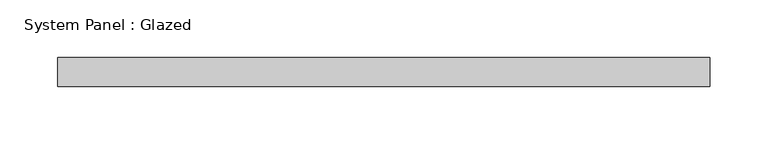
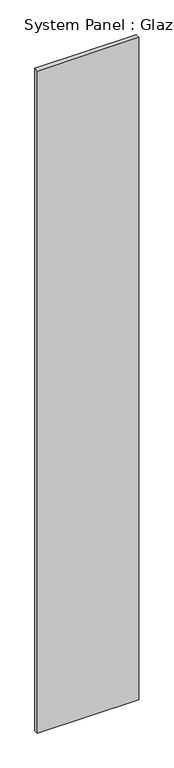
"""IFC4 building model written with IfcOpenShell, lengths in millimetres: plate geometry, System Panel : Glazed."""

from ifc_helpers import new_model, si_unit, origin, origin_with_axes, place, context, project, spatial, polyline, outline, extrude, source, transform, mapped, element, save


def system_panel_glazed_164e01dc(model_context):
    return source(origin(), model_context, "Body", "SweptSolid", [
        extrude(outline(polyline([(282.4999998, 24.5), (-282.4999998, 24.5), (-282.4999998, 49.5), (282.4999998, 49.5), (282.4999998, 24.5)])), origin_with_axes(), (0.0, 0.0, 1.0), 3900.0),
    ])


if __name__ == "__main__":
    model = new_model("IFC4")
    model_context = context("Model", 3, world=origin())
    ifc_project = project(units=[si_unit("LENGTHUNIT", "METRE", prefix="MILLI")], contexts=[model_context])
    site = spatial("IfcSite", under=ifc_project)
    building = spatial("IfcBuilding", under=site)
    placement = place(None, origin())
    system_panel_glazed_shape = system_panel_glazed_164e01dc(model_context)
    element("IfcPlate", 1, ObjectType="System Panel : Glazed", at=placement, inside=building, context=model_context, shape_type="MappedRepresentation", body=[
        mapped(system_panel_glazed_shape, transform((0.0, 0.0, 0.0), x_axis=(1.0, 0.0, 0.0), y_axis=(0.0, 1.0, 0.0), z_axis=(0.0, 0.0, 1.0))),
    ])
    save(model, "model.ifc")

# Revit data of these elements
# Type "System Panel : Glazed"
#   Keynote = "H11"
#   Construction Type Id = "GSP4R"
#   Analytic Construction = "1/8 in Pilkington single glazing"
#   Visual Light Transmittance = 0.9
#   Solar Heat Gain Coefficient = 0.86
#   Heat Transfer Coefficient (U) = 6.7069 W/(m²·K)
#   Define Thermal Properties by = 1
# Element 1 (IfcPlate, "System Panel : Glazed")
#   Materials on its faces: "Glass"
# Materials
#   "Glass": class "Glass", colour RGB 0 128 192, transparency 0.9, Description = "Soda Lime Glass", Cost = 0
